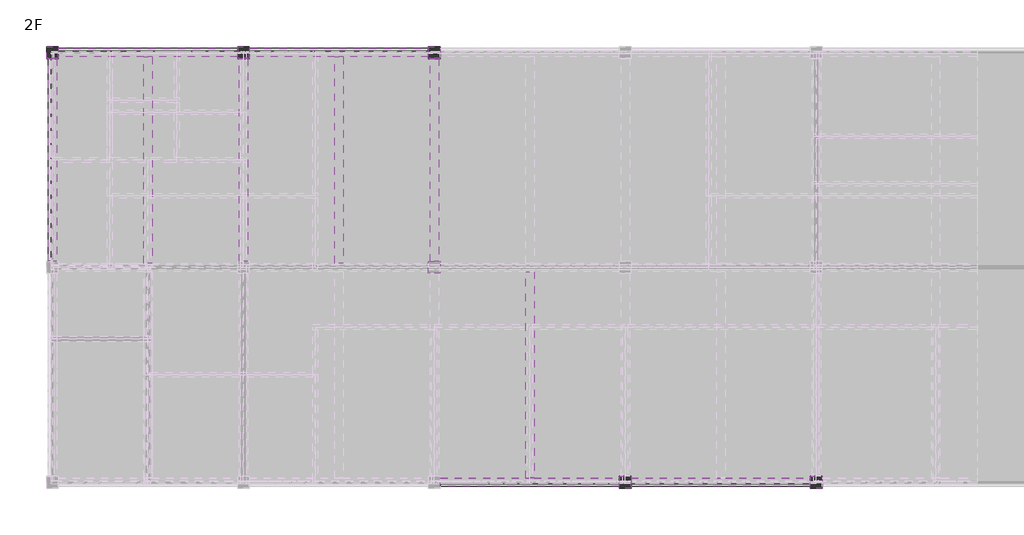
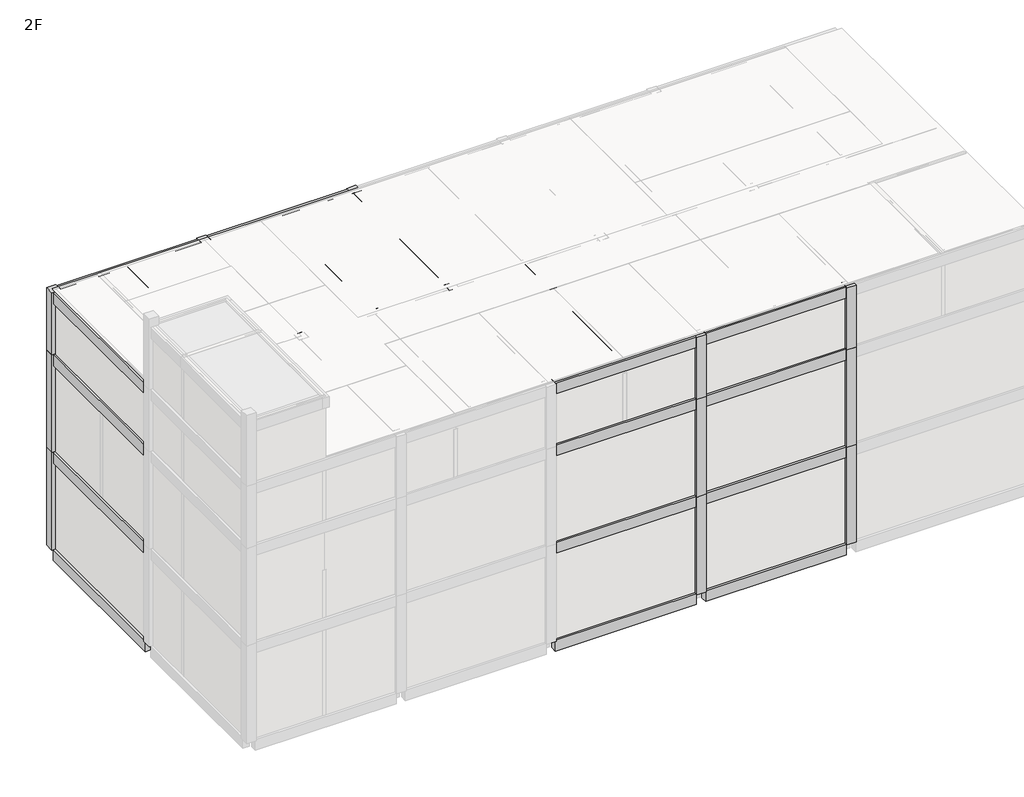
# One storey, part 5 of 7: 40 beams, 17 columns.
"""IFC4 building model written with IfcOpenShell, lengths in millimetres."""

from ifc_helpers import new_model, si_unit, frame, origin, place, context, project, spatial, polyline, outline, extrude, faceted_brep, element, save

model = new_model("IFC4")

# Units and contexts
model_context = context("Model", 3, world=origin())
ifc_project = project(units=[si_unit("LENGTHUNIT", "METRE", prefix="MILLI")], contexts=[model_context])

# Site, building, storey
site = spatial("IfcSite", under=ifc_project)
building = spatial("IfcBuilding", under=site)
storey = spatial("IfcBuildingStorey", under=building, Name="2F", Elevation=3500.0)

# Beams
placement = place(None, origin())
element("IfcBeam", 1, ObjectType="Concrete-Rectangular-Beam : BM111_400x500_RG1", at=placement, inside=storey, context=model_context, shape_type="SweptSolid", body=[
    extrude(outline(polyline([(49284.6521483, 181748.8614395), (49634.6521483, 181748.8614395), (49634.6521483, 173098.8614395), (49284.6521483, 173098.8614395), (49284.6521483, 181748.8614395)])), frame((0.0, 0.0, 2900.0), z_axis=(0.0, 0.0, 1.0), x_axis=(1.0, 0.0, 0.0)), (0.0, 0.0, 1.0), 600.0),
])
element("IfcBeam", 2, ObjectType="Concrete-Rectangular-Beam : BM111_400x500_RG1", at=placement, inside=storey, context=model_context, shape_type="SweptSolid", body=[
    extrude(outline(polyline([(57634.6521483, 173098.8614395), (57284.6521483, 173098.8614395), (57284.6521483, 181748.8614395), (57634.6521483, 181748.8614395), (57634.6521483, 173098.8614395)])), frame((0.0, 0.0, 2900.0), z_axis=(0.0, 0.0, 1.0), x_axis=(1.0, 0.0, 0.0)), (0.0, 0.0, 1.0), 600.0),
])
element("IfcBeam", 3, ObjectType="Concrete-Rectangular-Beam : BM111_400x500_RG1", at=placement, inside=storey, context=model_context, shape_type="SweptSolid", body=[
    extrude(outline(polyline([(65284.6521483, 172748.8614395), (65634.6521483, 172748.8614395), (65634.6521483, 164098.8614395), (65284.6521483, 164098.8614395), (65284.6521483, 172748.8614395)])), frame((0.0, 0.0, 2900.0), z_axis=(0.0, 0.0, 1.0), x_axis=(1.0, 0.0, 0.0)), (0.0, 0.0, 1.0), 600.0),
])
element("IfcBeam", 4, ObjectType="Concrete-Rectangular-Beam : BM111_400x500_RG1", at=placement, inside=storey, context=model_context, shape_type="SweptSolid", body=[
    extrude(outline(polyline([(49284.6521483, 181748.8614395), (49634.6521483, 181748.8614395), (49634.6521483, 173098.8614395), (49284.6521483, 173098.8614395), (49284.6521483, 181748.8614395)])), frame((0.0, 0.0, 8400.0), z_axis=(0.0, 0.0, 1.0), x_axis=(1.0, 0.0, 0.0)), (0.0, 0.0, 1.0), 600.0),
])
element("IfcBeam", 5, ObjectType="Concrete-Rectangular-Beam : BM111_400x500_RG1", at=placement, inside=storey, context=model_context, shape_type="SweptSolid", body=[
    extrude(outline(polyline([(57634.6521483, 173098.8614395), (57284.6521483, 173098.8614395), (57284.6521483, 181748.8614395), (57634.6521483, 181748.8614395), (57634.6521483, 173098.8614395)])), frame((0.0, 0.0, 8400.0), z_axis=(0.0, 0.0, 1.0), x_axis=(1.0, 0.0, 0.0)), (0.0, 0.0, 1.0), 600.0),
])
element("IfcBeam", 6, ObjectType="Concrete-Rectangular-Beam : BM111_400x500_RG1", at=placement, inside=storey, context=model_context, shape_type="SweptSolid", body=[
    extrude(outline(polyline([(65284.6521483, 172748.8614395), (65634.6521483, 172748.8614395), (65634.6521483, 164098.8614395), (65284.6521483, 164098.8614395), (65284.6521483, 172748.8614395)])), frame((0.0, 0.0, 8400.0), z_axis=(0.0, 0.0, 1.0), x_axis=(1.0, 0.0, 0.0)), (0.0, 0.0, 1.0), 600.0),
])
element("IfcBeam", 7, ObjectType="Concrete-Rectangular-Beam : BM111_400x500_RG1", at=placement, inside=storey, context=model_context, shape_type="SweptSolid", body=[
    extrude(outline(polyline([(49284.6521483, 181748.8614395), (49634.6521483, 181748.8614395), (49634.6521483, 173098.8614395), (49284.6521483, 173098.8614395), (49284.6521483, 181748.8614395)])), frame((0.0, 0.0, 13900.0), z_axis=(0.0, 0.0, 1.0), x_axis=(1.0, 0.0, 0.0)), (0.0, 0.0, 1.0), 600.0),
])
element("IfcBeam", 8, ObjectType="Concrete-Rectangular-Beam : BM111_400x500_RG1", at=placement, inside=storey, context=model_context, shape_type="SweptSolid", body=[
    extrude(outline(polyline([(57634.6521483, 173098.8614395), (57284.6521483, 173098.8614395), (57284.6521483, 181748.8614395), (57634.6521483, 181748.8614395), (57634.6521483, 173098.8614395)])), frame((0.0, 0.0, 13900.0), z_axis=(0.0, 0.0, 1.0), x_axis=(1.0, 0.0, 0.0)), (0.0, 0.0, 1.0), 600.0),
])
element("IfcBeam", 9, ObjectType="Concrete-Rectangular-Beam : BM111_400x500_RG1", at=placement, inside=storey, context=model_context, shape_type="SweptSolid", body=[
    extrude(outline(polyline([(65284.6521483, 172748.8614395), (65634.6521483, 172748.8614395), (65634.6521483, 164098.8614395), (65284.6521483, 164098.8614395), (65284.6521483, 172748.8614395)])), frame((0.0, 0.0, 13900.0), z_axis=(0.0, 0.0, 1.0), x_axis=(1.0, 0.0, 0.0)), (0.0, 0.0, 1.0), 600.0),
])
element("IfcBeam", 10, ObjectType="Concrete-Rectangular-Beam : BM111_400x500_RG1", at=placement, inside=storey, context=model_context, shape_type="SweptSolid", body=[
    extrude(outline(polyline([(49284.6521483, 181748.8614395), (49634.6521483, 181748.8614395), (49634.6521483, 173098.8614395), (49284.6521483, 173098.8614395), (49284.6521483, 181748.8614395)])), frame((0.0, 0.0, 17400.0), z_axis=(0.0, 0.0, 1.0), x_axis=(1.0, 0.0, 0.0)), (0.0, 0.0, 1.0), 600.0),
])
element("IfcBeam", 11, ObjectType="Concrete-Rectangular-Beam : BM111_400x500_RG1", at=placement, inside=storey, context=model_context, shape_type="SweptSolid", body=[
    extrude(outline(polyline([(57634.6521483, 173098.8614395), (57284.6521483, 173098.8614395), (57284.6521483, 181748.8614395), (57634.6521483, 181748.8614395), (57634.6521483, 173098.8614395)])), frame((0.0, 0.0, 17400.0), z_axis=(0.0, 0.0, 1.0), x_axis=(1.0, 0.0, 0.0)), (0.0, 0.0, 1.0), 600.0),
])
element("IfcBeam", 12, ObjectType="Concrete-Rectangular-Beam : BM111_400x500_RG1", at=placement, inside=storey, context=model_context, shape_type="SweptSolid", body=[
    extrude(outline(polyline([(65284.6521483, 172748.8614395), (65634.6521483, 172748.8614395), (65634.6521483, 164098.8614395), (65284.6521483, 164098.8614395), (65284.6521483, 172748.8614395)])), frame((0.0, 0.0, 17400.0), z_axis=(0.0, 0.0, 1.0), x_axis=(1.0, 0.0, 0.0)), (0.0, 0.0, 1.0), 600.0),
])
element("IfcBeam", 13, ObjectType="Concrete-Rectangular-Beam : BM111_400x500_RG1", at=placement, inside=storey, context=model_context, shape_type="Brep", body=[
    faceted_brep([(45709.6521483, 182098.8614395, 3500.0), (45709.6521483, 181748.8614395, 3500.0), (49284.6521483, 181748.8614395, 3500.0), (49634.6521483, 181748.8614395, 3500.0), (53209.6521483, 181748.8614395, 3500.0), (53209.6521483, 182098.8614395, 3500.0), (45709.6521483, 181748.8614395, 2900.0), (49284.6521483, 181748.8614395, 2900.0), (49634.6521483, 181748.8614395, 2900.0), (53209.6521483, 181748.8614395, 2900.0), (45709.6521483, 182098.8614395, 2900.0), (53209.6521483, 182098.8614395, 2900.0)], [[[0, 1, 2, 3, 4, 5]], [[1, 6, 7, 8, 9, 4, 3, 2]], [[6, 10, 11, 9, 8, 7]], [[10, 0, 5, 11]], [[1, 0, 10, 6]], [[5, 4, 9, 11]]]),
])
element("IfcBeam", 14, ObjectType="Concrete-Rectangular-Beam : BM111_400x500_RG1", at=placement, inside=storey, context=model_context, shape_type="Brep", body=[
    faceted_brep([(53709.6521483, 182098.8614395, 3500.0), (53709.6521483, 181748.8614395, 3500.0), (57284.6521483, 181748.8614395, 3500.0), (57634.6521483, 181748.8614395, 3500.0), (61209.6521483, 181748.8614395, 3500.0), (61209.6521483, 182098.8614395, 3500.0), (53709.6521483, 181748.8614395, 2900.0), (57284.6521483, 181748.8614395, 2900.0), (57634.6521483, 181748.8614395, 2900.0), (61209.6521483, 181748.8614395, 2900.0), (53709.6521483, 182098.8614395, 2900.0), (61209.6521483, 182098.8614395, 2900.0)], [[[0, 1, 2, 3, 4, 5]], [[1, 6, 7, 8, 9, 4, 3, 2]], [[6, 10, 11, 9, 8, 7]], [[10, 0, 5, 11]], [[1, 0, 10, 6]], [[5, 4, 9, 11]]]),
])
element("IfcBeam", 15, ObjectType="Concrete-Rectangular-Beam : BM111_400x500_RG1", at=placement, inside=storey, context=model_context, shape_type="Brep", body=[
    faceted_brep([(61709.6521483, 164098.8614395, 3500.0), (61709.6521483, 163748.8614395, 3500.0), (69209.6521483, 163748.8614395, 3500.0), (69209.6521483, 164098.8614395, 3500.0), (65634.6521483, 164098.8614395, 3500.0), (65284.6521483, 164098.8614395, 3500.0), (61709.6521483, 163748.8614395, 2900.0), (69209.6521483, 163748.8614395, 2900.0), (61709.6521483, 164098.8614395, 2900.0), (65284.6521483, 164098.8614395, 2900.0), (65634.6521483, 164098.8614395, 2900.0), (69209.6521483, 164098.8614395, 2900.0)], [[[0, 1, 2, 3, 4, 5]], [[1, 6, 7, 2]], [[6, 8, 9, 10, 11, 7]], [[8, 0, 5, 4, 3, 11, 10, 9]], [[1, 0, 8, 6]], [[3, 2, 7, 11]]]),
])
element("IfcBeam", 16, ObjectType="Concrete-Rectangular-Beam : BM111_400x500_RG1", at=placement, inside=storey, context=model_context, shape_type="Brep", body=[
    faceted_brep([(69709.6521483, 164098.8614395, 3500.0), (69709.6521483, 163748.8614395, 3500.0), (77209.6521483, 163748.8614395, 3500.0), (77209.6521483, 164098.8614395, 3500.0), (73634.6521483, 164098.8614395, 3500.0), (73284.6521483, 164098.8614395, 3500.0), (69709.6521483, 163748.8614395, 2900.0), (77209.6521483, 163748.8614395, 2900.0), (69709.6521483, 164098.8614395, 2900.0), (73284.6521483, 164098.8614395, 2900.0), (73634.6521483, 164098.8614395, 2900.0), (77209.6521483, 164098.8614395, 2900.0)], [[[0, 1, 2, 3, 4, 5]], [[1, 6, 7, 2]], [[6, 8, 9, 10, 11, 7]], [[8, 0, 5, 4, 3, 11, 10, 9]], [[1, 0, 8, 6]], [[3, 2, 7, 11]]]),
])
element("IfcBeam", 17, ObjectType="Concrete-Rectangular-Beam : BM111_400x500_RG1", at=placement, inside=storey, context=model_context, shape_type="Brep", body=[
    faceted_brep([(45709.6521483, 182098.8614395, 9000.0), (45709.6521483, 181748.8614395, 9000.0), (49284.6521483, 181748.8614395, 9000.0), (49634.6521483, 181748.8614395, 9000.0), (53209.6521483, 181748.8614395, 9000.0), (53209.6521483, 182098.8614395, 9000.0), (45709.6521483, 181748.8614395, 8400.0), (49284.6521483, 181748.8614395, 8400.0), (49634.6521483, 181748.8614395, 8400.0), (53209.6521483, 181748.8614395, 8400.0), (45709.6521483, 182098.8614395, 8400.0), (53209.6521483, 182098.8614395, 8400.0)], [[[0, 1, 2, 3, 4, 5]], [[1, 6, 7, 8, 9, 4, 3, 2]], [[6, 10, 11, 9, 8, 7]], [[10, 0, 5, 11]], [[1, 0, 10, 6]], [[5, 4, 9, 11]]]),
])
element("IfcBeam", 18, ObjectType="Concrete-Rectangular-Beam : BM111_400x500_RG1", at=placement, inside=storey, context=model_context, shape_type="Brep", body=[
    faceted_brep([(53709.6521483, 182098.8614395, 9000.0), (53709.6521483, 181748.8614395, 9000.0), (57284.6521483, 181748.8614395, 9000.0), (57634.6521483, 181748.8614395, 9000.0), (61209.6521483, 181748.8614395, 9000.0), (61209.6521483, 182098.8614395, 9000.0), (53709.6521483, 181748.8614395, 8400.0), (57284.6521483, 181748.8614395, 8400.0), (57634.6521483, 181748.8614395, 8400.0), (61209.6521483, 181748.8614395, 8400.0), (53709.6521483, 182098.8614395, 8400.0), (61209.6521483, 182098.8614395, 8400.0)], [[[0, 1, 2, 3, 4, 5]], [[1, 6, 7, 8, 9, 4, 3, 2]], [[6, 10, 11, 9, 8, 7]], [[10, 0, 5, 11]], [[1, 0, 10, 6]], [[5, 4, 9, 11]]]),
])
element("IfcBeam", 19, ObjectType="Concrete-Rectangular-Beam : BM111_400x500_RG1", at=placement, inside=storey, context=model_context, shape_type="Brep", body=[
    faceted_brep([(61709.6521483, 164098.8614395, 9000.0), (61709.6521483, 163748.8614395, 9000.0), (69209.6521483, 163748.8614395, 9000.0), (69209.6521483, 164098.8614395, 9000.0), (65634.6521483, 164098.8614395, 9000.0), (65284.6521483, 164098.8614395, 9000.0), (61709.6521483, 163748.8614395, 8400.0), (69209.6521483, 163748.8614395, 8400.0), (61709.6521483, 164098.8614395, 8400.0), (65284.6521483, 164098.8614395, 8400.0), (65634.6521483, 164098.8614395, 8400.0), (69209.6521483, 164098.8614395, 8400.0)], [[[0, 1, 2, 3, 4, 5]], [[1, 6, 7, 2]], [[6, 8, 9, 10, 11, 7]], [[8, 0, 5, 4, 3, 11, 10, 9]], [[1, 0, 8, 6]], [[3, 2, 7, 11]]]),
])
element("IfcBeam", 20, ObjectType="Concrete-Rectangular-Beam : BM111_400x500_RG1", at=placement, inside=storey, context=model_context, shape_type="Brep", body=[
    faceted_brep([(69709.6521483, 164098.8614395, 9000.0), (69709.6521483, 163748.8614395, 9000.0), (77209.6521483, 163748.8614395, 9000.0), (77209.6521483, 164098.8614395, 9000.0), (73634.6521483, 164098.8614395, 9000.0), (73284.6521483, 164098.8614395, 9000.0), (69709.6521483, 163748.8614395, 8400.0), (77209.6521483, 163748.8614395, 8400.0), (69709.6521483, 164098.8614395, 8400.0), (73284.6521483, 164098.8614395, 8400.0), (73634.6521483, 164098.8614395, 8400.0), (77209.6521483, 164098.8614395, 8400.0)], [[[0, 1, 2, 3, 4, 5]], [[1, 6, 7, 2]], [[6, 8, 9, 10, 11, 7]], [[8, 0, 5, 4, 3, 11, 10, 9]], [[1, 0, 8, 6]], [[3, 2, 7, 11]]]),
])
element("IfcBeam", 21, ObjectType="Concrete-Rectangular-Beam : BM111_400x500_RG1", at=placement, inside=storey, context=model_context, shape_type="Brep", body=[
    faceted_brep([(45709.6521483, 182098.8614395, 14500.0), (45709.6521483, 181748.8614395, 14500.0), (49284.6521483, 181748.8614395, 14500.0), (49634.6521483, 181748.8614395, 14500.0), (53209.6521483, 181748.8614395, 14500.0), (53209.6521483, 182098.8614395, 14500.0), (45709.6521483, 181748.8614395, 13900.0), (49284.6521483, 181748.8614395, 13900.0), (49634.6521483, 181748.8614395, 13900.0), (53209.6521483, 181748.8614395, 13900.0), (45709.6521483, 182098.8614395, 13900.0), (53209.6521483, 182098.8614395, 13900.0)], [[[0, 1, 2, 3, 4, 5]], [[1, 6, 7, 8, 9, 4, 3, 2]], [[6, 10, 11, 9, 8, 7]], [[10, 0, 5, 11]], [[1, 0, 10, 6]], [[5, 4, 9, 11]]]),
])
element("IfcBeam", 22, ObjectType="Concrete-Rectangular-Beam : BM111_400x500_RG1", at=placement, inside=storey, context=model_context, shape_type="Brep", body=[
    faceted_brep([(53709.6521483, 182098.8614395, 14500.0), (53709.6521483, 181748.8614395, 14500.0), (57284.6521483, 181748.8614395, 14500.0), (57634.6521483, 181748.8614395, 14500.0), (61209.6521483, 181748.8614395, 14500.0), (61209.6521483, 182098.8614395, 14500.0), (53709.6521483, 181748.8614395, 13900.0), (57284.6521483, 181748.8614395, 13900.0), (57634.6521483, 181748.8614395, 13900.0), (61209.6521483, 181748.8614395, 13900.0), (53709.6521483, 182098.8614395, 13900.0), (61209.6521483, 182098.8614395, 13900.0)], [[[0, 1, 2, 3, 4, 5]], [[1, 6, 7, 8, 9, 4, 3, 2]], [[6, 10, 11, 9, 8, 7]], [[10, 0, 5, 11]], [[1, 0, 10, 6]], [[5, 4, 9, 11]]]),
])
element("IfcBeam", 23, ObjectType="Concrete-Rectangular-Beam : BM111_400x500_RG1", at=placement, inside=storey, context=model_context, shape_type="Brep", body=[
    faceted_brep([(61709.6521483, 164098.8614395, 14500.0), (61709.6521483, 163748.8614395, 14500.0), (69209.6521483, 163748.8614395, 14500.0), (69209.6521483, 164098.8614395, 14500.0), (65634.6521483, 164098.8614395, 14500.0), (65284.6521483, 164098.8614395, 14500.0), (61709.6521483, 163748.8614395, 13900.0), (69209.6521483, 163748.8614395, 13900.0), (61709.6521483, 164098.8614395, 13900.0), (65284.6521483, 164098.8614395, 13900.0), (65634.6521483, 164098.8614395, 13900.0), (69209.6521483, 164098.8614395, 13900.0)], [[[0, 1, 2, 3, 4, 5]], [[1, 6, 7, 2]], [[6, 8, 9, 10, 11, 7]], [[8, 0, 5, 4, 3, 11, 10, 9]], [[1, 0, 8, 6]], [[3, 2, 7, 11]]]),
])
element("IfcBeam", 24, ObjectType="Concrete-Rectangular-Beam : BM111_400x500_RG1", at=placement, inside=storey, context=model_context, shape_type="Brep", body=[
    faceted_brep([(69709.6521483, 164098.8614395, 14500.0), (69709.6521483, 163748.8614395, 14500.0), (77209.6521483, 163748.8614395, 14500.0), (77209.6521483, 164098.8614395, 14500.0), (73634.6521483, 164098.8614395, 14500.0), (73284.6521483, 164098.8614395, 14500.0), (69709.6521483, 163748.8614395, 13900.0), (77209.6521483, 163748.8614395, 13900.0), (69709.6521483, 164098.8614395, 13900.0), (73284.6521483, 164098.8614395, 13900.0), (73634.6521483, 164098.8614395, 13900.0), (77209.6521483, 164098.8614395, 13900.0)], [[[0, 1, 2, 3, 4, 5]], [[1, 6, 7, 2]], [[6, 8, 9, 10, 11, 7]], [[8, 0, 5, 4, 3, 11, 10, 9]], [[1, 0, 8, 6]], [[3, 2, 7, 11]]]),
])
element("IfcBeam", 25, ObjectType="Concrete-Rectangular-Beam : BM111_400x500_RG1", at=placement, inside=storey, context=model_context, shape_type="Brep", body=[
    faceted_brep([(45709.6521483, 182098.8614395, 18000.0), (45709.6521483, 181748.8614395, 18000.0), (49284.6521483, 181748.8614395, 18000.0), (49634.6521483, 181748.8614395, 18000.0), (53209.6521483, 181748.8614395, 18000.0), (53209.6521483, 182098.8614395, 18000.0), (45709.6521483, 181748.8614395, 17400.0), (49284.6521483, 181748.8614395, 17400.0), (49634.6521483, 181748.8614395, 17400.0), (53209.6521483, 181748.8614395, 17400.0), (45709.6521483, 182098.8614395, 17400.0), (53209.6521483, 182098.8614395, 17400.0)], [[[0, 1, 2, 3, 4, 5]], [[1, 6, 7, 8, 9, 4, 3, 2]], [[6, 10, 11, 9, 8, 7]], [[10, 0, 5, 11]], [[1, 0, 10, 6]], [[5, 4, 9, 11]]]),
])
element("IfcBeam", 26, ObjectType="Concrete-Rectangular-Beam : BM111_400x500_RG1", at=placement, inside=storey, context=model_context, shape_type="Brep", body=[
    faceted_brep([(53709.6521483, 182098.8614395, 18000.0), (53709.6521483, 181748.8614395, 18000.0), (57284.6521483, 181748.8614395, 18000.0), (57634.6521483, 181748.8614395, 18000.0), (61209.6521483, 181748.8614395, 18000.0), (61209.6521483, 182098.8614395, 18000.0), (53709.6521483, 181748.8614395, 17400.0), (57284.6521483, 181748.8614395, 17400.0), (57634.6521483, 181748.8614395, 17400.0), (61209.6521483, 181748.8614395, 17400.0), (53709.6521483, 182098.8614395, 17400.0), (61209.6521483, 182098.8614395, 17400.0)], [[[0, 1, 2, 3, 4, 5]], [[1, 6, 7, 8, 9, 4, 3, 2]], [[6, 10, 11, 9, 8, 7]], [[10, 0, 5, 11]], [[1, 0, 10, 6]], [[5, 4, 9, 11]]]),
])
element("IfcBeam", 27, ObjectType="Concrete-Rectangular-Beam : BM111_400x500_RG1", at=placement, inside=storey, context=model_context, shape_type="Brep", body=[
    faceted_brep([(61709.6521483, 164098.8614395, 18000.0), (61709.6521483, 163748.8614395, 18000.0), (69209.6521483, 163748.8614395, 18000.0), (69209.6521483, 164098.8614395, 18000.0), (65634.6521483, 164098.8614395, 18000.0), (65284.6521483, 164098.8614395, 18000.0), (61709.6521483, 163748.8614395, 17400.0), (69209.6521483, 163748.8614395, 17400.0), (61709.6521483, 164098.8614395, 17400.0), (65284.6521483, 164098.8614395, 17400.0), (65634.6521483, 164098.8614395, 17400.0), (69209.6521483, 164098.8614395, 17400.0)], [[[0, 1, 2, 3, 4, 5]], [[1, 6, 7, 2]], [[6, 8, 9, 10, 11, 7]], [[8, 0, 5, 4, 3, 11, 10, 9]], [[1, 0, 8, 6]], [[3, 2, 7, 11]]]),
])
element("IfcBeam", 28, ObjectType="Concrete-Rectangular-Beam : BM111_400x500_RG1", at=placement, inside=storey, context=model_context, shape_type="Brep", body=[
    faceted_brep([(69709.6521483, 164098.8614395, 18000.0), (69709.6521483, 163748.8614395, 18000.0), (77209.6521483, 163748.8614395, 18000.0), (77209.6521483, 164098.8614395, 18000.0), (73634.6521483, 164098.8614395, 18000.0), (73284.6521483, 164098.8614395, 18000.0), (69709.6521483, 163748.8614395, 17400.0), (77209.6521483, 163748.8614395, 17400.0), (69709.6521483, 164098.8614395, 17400.0), (73284.6521483, 164098.8614395, 17400.0), (73634.6521483, 164098.8614395, 17400.0), (77209.6521483, 164098.8614395, 17400.0)], [[[0, 1, 2, 3, 4, 5]], [[1, 6, 7, 2]], [[6, 8, 9, 10, 11, 7]], [[8, 0, 5, 4, 3, 11, 10, 9]], [[1, 0, 8, 6]], [[3, 2, 7, 11]]]),
])
element("IfcBeam", 29, ObjectType="Concrete-Rectangular-Beam : BM111_400x500_RG1", at=placement, inside=storey, context=model_context, shape_type="SweptSolid", body=[
    extrude(outline(polyline([(45284.6521483, 181673.8614395), (45634.6521483, 181673.8614395), (45634.6521483, 173173.8614395), (45284.6521483, 173173.8614395), (45284.6521483, 181673.8614395)])), frame((0.0, 0.0, 2900.0), z_axis=(0.0, 0.0, 1.0), x_axis=(1.0, 0.0, 0.0)), (0.0, 0.0, 1.0), 600.0),
])
element("IfcBeam", 30, ObjectType="Concrete-Rectangular-Beam : BM111_400x500_RG1", at=placement, inside=storey, context=model_context, shape_type="SweptSolid", body=[
    extrude(outline(polyline([(53284.6521483, 181673.8614395), (53634.6521483, 181673.8614395), (53634.6521483, 173173.8614395), (53284.6521483, 173173.8614395), (53284.6521483, 181673.8614395)])), frame((0.0, 0.0, 2900.0), z_axis=(0.0, 0.0, 1.0), x_axis=(1.0, 0.0, 0.0)), (0.0, 0.0, 1.0), 600.0),
])
element("IfcBeam", 31, ObjectType="Concrete-Rectangular-Beam : BM111_400x500_RG1", at=placement, inside=storey, context=model_context, shape_type="SweptSolid", body=[
    extrude(outline(polyline([(61284.6521483, 181673.8614395), (61634.6521483, 181673.8614395), (61634.6521483, 173173.8614395), (61284.6521483, 173173.8614395), (61284.6521483, 181673.8614395)])), frame((0.0, 0.0, 2900.0), z_axis=(0.0, 0.0, 1.0), x_axis=(1.0, 0.0, 0.0)), (0.0, 0.0, 1.0), 600.0),
])
element("IfcBeam", 32, ObjectType="Concrete-Rectangular-Beam : BM111_400x500_RG1", at=placement, inside=storey, context=model_context, shape_type="SweptSolid", body=[
    extrude(outline(polyline([(45284.6521483, 181673.8614395), (45634.6521483, 181673.8614395), (45634.6521483, 173173.8614395), (45284.6521483, 173173.8614395), (45284.6521483, 181673.8614395)])), frame((0.0, 0.0, 8400.0), z_axis=(0.0, 0.0, 1.0), x_axis=(1.0, 0.0, 0.0)), (0.0, 0.0, 1.0), 600.0),
])
element("IfcBeam", 33, ObjectType="Concrete-Rectangular-Beam : BM111_400x500_RG1", at=placement, inside=storey, context=model_context, shape_type="SweptSolid", body=[
    extrude(outline(polyline([(53284.6521483, 181673.8614395), (53634.6521483, 181673.8614395), (53634.6521483, 173173.8614395), (53284.6521483, 173173.8614395), (53284.6521483, 181673.8614395)])), frame((0.0, 0.0, 8400.0), z_axis=(0.0, 0.0, 1.0), x_axis=(1.0, 0.0, 0.0)), (0.0, 0.0, 1.0), 600.0),
])
element("IfcBeam", 34, ObjectType="Concrete-Rectangular-Beam : BM111_400x500_RG1", at=placement, inside=storey, context=model_context, shape_type="SweptSolid", body=[
    extrude(outline(polyline([(61284.6521483, 181673.8614395), (61634.6521483, 181673.8614395), (61634.6521483, 173173.8614395), (61284.6521483, 173173.8614395), (61284.6521483, 181673.8614395)])), frame((0.0, 0.0, 8400.0), z_axis=(0.0, 0.0, 1.0), x_axis=(1.0, 0.0, 0.0)), (0.0, 0.0, 1.0), 600.0),
])
element("IfcBeam", 35, ObjectType="Concrete-Rectangular-Beam : BM111_400x500_RG1", at=placement, inside=storey, context=model_context, shape_type="SweptSolid", body=[
    extrude(outline(polyline([(45284.6521483, 181673.8614395), (45634.6521483, 181673.8614395), (45634.6521483, 173173.8614395), (45284.6521483, 173173.8614395), (45284.6521483, 181673.8614395)])), frame((0.0, 0.0, 13900.0), z_axis=(0.0, 0.0, 1.0), x_axis=(1.0, 0.0, 0.0)), (0.0, 0.0, 1.0), 600.0),
])
element("IfcBeam", 36, ObjectType="Concrete-Rectangular-Beam : BM111_400x500_RG1", at=placement, inside=storey, context=model_context, shape_type="SweptSolid", body=[
    extrude(outline(polyline([(53284.6521483, 181673.8614395), (53634.6521483, 181673.8614395), (53634.6521483, 173173.8614395), (53284.6521483, 173173.8614395), (53284.6521483, 181673.8614395)])), frame((0.0, 0.0, 13900.0), z_axis=(0.0, 0.0, 1.0), x_axis=(1.0, 0.0, 0.0)), (0.0, 0.0, 1.0), 600.0),
])
element("IfcBeam", 37, ObjectType="Concrete-Rectangular-Beam : BM111_400x500_RG1", at=placement, inside=storey, context=model_context, shape_type="SweptSolid", body=[
    extrude(outline(polyline([(61284.6521483, 181673.8614395), (61634.6521483, 181673.8614395), (61634.6521483, 173173.8614395), (61284.6521483, 173173.8614395), (61284.6521483, 181673.8614395)])), frame((0.0, 0.0, 13900.0), z_axis=(0.0, 0.0, 1.0), x_axis=(1.0, 0.0, 0.0)), (0.0, 0.0, 1.0), 600.0),
])
element("IfcBeam", 38, ObjectType="Concrete-Rectangular-Beam : BM111_400x500_RG1", at=placement, inside=storey, context=model_context, shape_type="SweptSolid", body=[
    extrude(outline(polyline([(45284.6521483, 181673.8614395), (45634.6521483, 181673.8614395), (45634.6521483, 173173.8614395), (45284.6521483, 173173.8614395), (45284.6521483, 181673.8614395)])), frame((0.0, 0.0, 17400.0), z_axis=(0.0, 0.0, 1.0), x_axis=(1.0, 0.0, 0.0)), (0.0, 0.0, 1.0), 600.0),
])
element("IfcBeam", 39, ObjectType="Concrete-Rectangular-Beam : BM111_400x500_RG1", at=placement, inside=storey, context=model_context, shape_type="SweptSolid", body=[
    extrude(outline(polyline([(53284.6521483, 181673.8614395), (53634.6521483, 181673.8614395), (53634.6521483, 173173.8614395), (53284.6521483, 173173.8614395), (53284.6521483, 181673.8614395)])), frame((0.0, 0.0, 17400.0), z_axis=(0.0, 0.0, 1.0), x_axis=(1.0, 0.0, 0.0)), (0.0, 0.0, 1.0), 600.0),
])
element("IfcBeam", 40, ObjectType="Concrete-Rectangular-Beam : BM111_400x500_RG1", at=placement, inside=storey, context=model_context, shape_type="SweptSolid", body=[
    extrude(outline(polyline([(61284.6521483, 181673.8614395), (61634.6521483, 181673.8614395), (61634.6521483, 173173.8614395), (61284.6521483, 173173.8614395), (61284.6521483, 181673.8614395)])), frame((0.0, 0.0, 17400.0), z_axis=(0.0, 0.0, 1.0), x_axis=(1.0, 0.0, 0.0)), (0.0, 0.0, 1.0), 600.0),
])

# Columns
element("IfcColumn", 41, ObjectType="Concrete-Rectangular-Column : CL111_500x500", at=placement, inside=storey, context=model_context, shape_type="Brep", body=[
    faceted_brep([(45709.6521483, 182173.8614395, 3500.0), (45709.6521483, 181673.8614395, 3500.0), (45209.6521483, 181673.8614395, 3500.0), (45209.6521483, 182173.8614395, 3500.0), (45709.6521483, 182173.8614395, 9000.0), (45709.6521483, 182098.8614395, 9000.0), (45709.6521483, 181748.8614395, 9000.0), (45709.6521483, 181673.8614395, 9000.0), (45634.6521483, 181673.8614395, 9000.0), (45284.6521483, 181673.8614395, 9000.0), (45209.6521483, 181673.8614395, 9000.0), (45209.6521483, 182173.8614395, 9000.0)], [[[0, 1, 2, 3]], [[4, 5, 6, 7, 1, 0]], [[7, 8, 9, 10, 2, 1]], [[10, 11, 3, 2]], [[11, 4, 0, 3]], [[4, 11, 10, 9, 8, 7, 6, 5]]]),
])
element("IfcColumn", 42, ObjectType="Concrete-Rectangular-Column : CL111_500x500", at=placement, inside=storey, context=model_context, shape_type="Brep", body=[
    faceted_brep([(45709.6521483, 182173.8614395, 9000.0), (45709.6521483, 181673.8614395, 9000.0), (45209.6521483, 181673.8614395, 9000.0), (45209.6521483, 182173.8614395, 9000.0), (45709.6521483, 182173.8614395, 14500.0), (45709.6521483, 182098.8614395, 14500.0), (45709.6521483, 181748.8614395, 14500.0), (45709.6521483, 181673.8614395, 14500.0), (45634.6521483, 181673.8614395, 14500.0), (45284.6521483, 181673.8614395, 14500.0), (45209.6521483, 181673.8614395, 14500.0), (45209.6521483, 182173.8614395, 14500.0)], [[[0, 1, 2, 3]], [[4, 5, 6, 7, 1, 0]], [[7, 8, 9, 10, 2, 1]], [[10, 11, 3, 2]], [[11, 4, 0, 3]], [[4, 11, 10, 9, 8, 7, 6, 5]]]),
])
element("IfcColumn", 43, ObjectType="Concrete-Rectangular-Column : CL111_500x500", at=placement, inside=storey, context=model_context, shape_type="Brep", body=[
    faceted_brep([(45709.6521483, 182173.8614395, 14500.0), (45709.6521483, 181673.8614395, 14500.0), (45209.6521483, 181673.8614395, 14500.0), (45209.6521483, 182173.8614395, 14500.0), (45709.6521483, 182173.8614395, 18000.0), (45709.6521483, 182098.8614395, 18000.0), (45709.6521483, 181748.8614395, 18000.0), (45709.6521483, 181673.8614395, 18000.0), (45634.6521483, 181673.8614395, 18000.0), (45284.6521483, 181673.8614395, 18000.0), (45209.6521483, 181673.8614395, 18000.0), (45209.6521483, 182173.8614395, 18000.0)], [[[0, 1, 2, 3]], [[4, 5, 6, 7, 1, 0]], [[7, 8, 9, 10, 2, 1]], [[10, 11, 3, 2]], [[11, 4, 0, 3]], [[4, 11, 10, 9, 8, 7, 6, 5]]]),
])
element("IfcColumn", 44, ObjectType="Concrete-Rectangular-Column : CL111_500x500", at=placement, inside=storey, context=model_context, shape_type="Brep", body=[
    faceted_brep([(53709.6521483, 182173.8614395, 3500.0), (53709.6521483, 181673.8614395, 3500.0), (53209.6521483, 181673.8614395, 3500.0), (53209.6521483, 182173.8614395, 3500.0), (53709.6521483, 182173.8614395, 9000.0), (53709.6521483, 182098.8614395, 9000.0), (53709.6521483, 181748.8614395, 9000.0), (53709.6521483, 181673.8614395, 9000.0), (53634.6521483, 181673.8614395, 9000.0), (53284.6521483, 181673.8614395, 9000.0), (53209.6521483, 181673.8614395, 9000.0), (53209.6521483, 181748.8614395, 9000.0), (53209.6521483, 182098.8614395, 9000.0), (53209.6521483, 182173.8614395, 9000.0)], [[[0, 1, 2, 3]], [[4, 5, 6, 7, 1, 0]], [[7, 8, 9, 10, 2, 1]], [[10, 11, 12, 13, 3, 2]], [[13, 4, 0, 3]], [[4, 13, 12, 11, 10, 9, 8, 7, 6, 5]]]),
])
element("IfcColumn", 45, ObjectType="Concrete-Rectangular-Column : CL111_500x500", at=placement, inside=storey, context=model_context, shape_type="Brep", body=[
    faceted_brep([(53709.6521483, 182173.8614395, 9000.0), (53709.6521483, 181673.8614395, 9000.0), (53209.6521483, 181673.8614395, 9000.0), (53209.6521483, 182173.8614395, 9000.0), (53709.6521483, 182173.8614395, 14500.0), (53709.6521483, 182098.8614395, 14500.0), (53709.6521483, 181748.8614395, 14500.0), (53709.6521483, 181673.8614395, 14500.0), (53634.6521483, 181673.8614395, 14500.0), (53284.6521483, 181673.8614395, 14500.0), (53209.6521483, 181673.8614395, 14500.0), (53209.6521483, 181748.8614395, 14500.0), (53209.6521483, 182098.8614395, 14500.0), (53209.6521483, 182173.8614395, 14500.0)], [[[0, 1, 2, 3]], [[4, 5, 6, 7, 1, 0]], [[7, 8, 9, 10, 2, 1]], [[10, 11, 12, 13, 3, 2]], [[13, 4, 0, 3]], [[4, 13, 12, 11, 10, 9, 8, 7, 6, 5]]]),
])
element("IfcColumn", 46, ObjectType="Concrete-Rectangular-Column : CL111_500x500", at=placement, inside=storey, context=model_context, shape_type="Brep", body=[
    faceted_brep([(53709.6521483, 182173.8614395, 14500.0), (53709.6521483, 181673.8614395, 14500.0), (53209.6521483, 181673.8614395, 14500.0), (53209.6521483, 182173.8614395, 14500.0), (53709.6521483, 182173.8614395, 18000.0), (53709.6521483, 182098.8614395, 18000.0), (53709.6521483, 181748.8614395, 18000.0), (53709.6521483, 181673.8614395, 18000.0), (53634.6521483, 181673.8614395, 18000.0), (53284.6521483, 181673.8614395, 18000.0), (53209.6521483, 181673.8614395, 18000.0), (53209.6521483, 181748.8614395, 18000.0), (53209.6521483, 182098.8614395, 18000.0), (53209.6521483, 182173.8614395, 18000.0)], [[[0, 1, 2, 3]], [[4, 5, 6, 7, 1, 0]], [[7, 8, 9, 10, 2, 1]], [[10, 11, 12, 13, 3, 2]], [[13, 4, 0, 3]], [[4, 13, 12, 11, 10, 9, 8, 7, 6, 5]]]),
])
element("IfcColumn", 47, ObjectType="Concrete-Rectangular-Column : CL111_500x500", at=placement, inside=storey, context=model_context, shape_type="Brep", body=[
    faceted_brep([(61709.6521483, 182173.8614395, 3500.0), (61709.6521483, 181673.8614395, 3500.0), (61209.6521483, 181673.8614395, 3500.0), (61209.6521483, 182173.8614395, 3500.0), (61709.6521483, 182173.8614395, 9000.0), (61709.6521483, 182098.8614395, 9000.0), (61709.6521483, 181748.8614395, 9000.0), (61709.6521483, 181673.8614395, 9000.0), (61634.6521483, 181673.8614395, 9000.0), (61284.6521483, 181673.8614395, 9000.0), (61209.6521483, 181673.8614395, 9000.0), (61209.6521483, 181748.8614395, 9000.0), (61209.6521483, 182098.8614395, 9000.0), (61209.6521483, 182173.8614395, 9000.0)], [[[0, 1, 2, 3]], [[4, 5, 6, 7, 1, 0]], [[7, 8, 9, 10, 2, 1]], [[10, 11, 12, 13, 3, 2]], [[13, 4, 0, 3]], [[4, 13, 12, 11, 10, 9, 8, 7, 6, 5]]]),
])
element("IfcColumn", 48, ObjectType="Concrete-Rectangular-Column : CL111_500x500", at=placement, inside=storey, context=model_context, shape_type="Brep", body=[
    faceted_brep([(61709.6521483, 182173.8614395, 9000.0), (61709.6521483, 181673.8614395, 9000.0), (61209.6521483, 181673.8614395, 9000.0), (61209.6521483, 182173.8614395, 9000.0), (61709.6521483, 182173.8614395, 14500.0), (61709.6521483, 182098.8614395, 14500.0), (61709.6521483, 181748.8614395, 14500.0), (61709.6521483, 181673.8614395, 14500.0), (61634.6521483, 181673.8614395, 14500.0), (61284.6521483, 181673.8614395, 14500.0), (61209.6521483, 181673.8614395, 14500.0), (61209.6521483, 181748.8614395, 14500.0), (61209.6521483, 182098.8614395, 14500.0), (61209.6521483, 182173.8614395, 14500.0)], [[[0, 1, 2, 3]], [[4, 5, 6, 7, 1, 0]], [[7, 8, 9, 10, 2, 1]], [[10, 11, 12, 13, 3, 2]], [[13, 4, 0, 3]], [[4, 13, 12, 11, 10, 9, 8, 7, 6, 5]]]),
])
element("IfcColumn", 49, ObjectType="Concrete-Rectangular-Column : CL111_500x500", at=placement, inside=storey, context=model_context, shape_type="Brep", body=[
    faceted_brep([(61709.6521483, 182173.8614395, 14500.0), (61709.6521483, 181673.8614395, 14500.0), (61209.6521483, 181673.8614395, 14500.0), (61209.6521483, 182173.8614395, 14500.0), (61709.6521483, 182173.8614395, 18000.0), (61709.6521483, 182098.8614395, 18000.0), (61709.6521483, 181748.8614395, 18000.0), (61709.6521483, 181673.8614395, 18000.0), (61634.6521483, 181673.8614395, 18000.0), (61284.6521483, 181673.8614395, 18000.0), (61209.6521483, 181673.8614395, 18000.0), (61209.6521483, 181748.8614395, 18000.0), (61209.6521483, 182098.8614395, 18000.0), (61209.6521483, 182173.8614395, 18000.0)], [[[0, 1, 2, 3]], [[4, 5, 6, 7, 1, 0]], [[7, 8, 9, 10, 2, 1]], [[10, 11, 12, 13, 3, 2]], [[13, 4, 0, 3]], [[4, 13, 12, 11, 10, 9, 8, 7, 6, 5]]]),
])
element("IfcColumn", 50, ObjectType="Concrete-Rectangular-Column : CL111_500x500", at=placement, inside=storey, context=model_context, shape_type="Brep", body=[
    faceted_brep([(61709.6521483, 173173.8614395, 9000.0), (61709.6521483, 172673.8614395, 9000.0), (61209.6521483, 172673.8614395, 9000.0), (61209.6521483, 173173.8614395, 9000.0), (61709.6521483, 173173.8614395, 14500.0), (61709.6521483, 173098.8614395, 14500.0), (61709.6521483, 172748.8614395, 14500.0), (61709.6521483, 172673.8614395, 14500.0), (61634.6521483, 172673.8614395, 14500.0), (61284.6521483, 172673.8614395, 14500.0), (61209.6521483, 172673.8614395, 14500.0), (61209.6521483, 172748.8614395, 14500.0), (61209.6521483, 173098.8614395, 14500.0), (61209.6521483, 173173.8614395, 14500.0), (61284.6521483, 173173.8614395, 14500.0), (61634.6521483, 173173.8614395, 14500.0)], [[[0, 1, 2, 3]], [[4, 5, 6, 7, 1, 0]], [[7, 8, 9, 10, 2, 1]], [[10, 11, 12, 13, 3, 2]], [[13, 14, 15, 4, 0, 3]], [[4, 15, 14, 13, 12, 11, 10, 9, 8, 7, 6, 5]]]),
])
element("IfcColumn", 51, ObjectType="Concrete-Rectangular-Column : CL111_500x500", at=placement, inside=storey, context=model_context, shape_type="Brep", body=[
    faceted_brep([(61709.6521483, 173173.8614395, 14500.0), (61709.6521483, 172673.8614395, 14500.0), (61209.6521483, 172673.8614395, 14500.0), (61209.6521483, 173173.8614395, 14500.0), (61709.6521483, 173173.8614395, 18000.0), (61709.6521483, 173098.8614395, 18000.0), (61709.6521483, 172748.8614395, 18000.0), (61709.6521483, 172673.8614395, 18000.0), (61634.6521483, 172673.8614395, 18000.0), (61284.6521483, 172673.8614395, 18000.0), (61209.6521483, 172673.8614395, 18000.0), (61209.6521483, 172748.8614395, 18000.0), (61209.6521483, 173098.8614395, 18000.0), (61209.6521483, 173173.8614395, 18000.0), (61284.6521483, 173173.8614395, 18000.0), (61634.6521483, 173173.8614395, 18000.0)], [[[0, 1, 2, 3]], [[4, 5, 6, 7, 1, 0]], [[7, 8, 9, 10, 2, 1]], [[10, 11, 12, 13, 3, 2]], [[13, 14, 15, 4, 0, 3]], [[4, 15, 14, 13, 12, 11, 10, 9, 8, 7, 6, 5]]]),
])
element("IfcColumn", 52, ObjectType="Concrete-Rectangular-Column : CL111_500x500", at=placement, inside=storey, context=model_context, shape_type="Brep", body=[
    faceted_brep([(69709.6521483, 164173.8614395, 3500.0), (69709.6521483, 163673.8614395, 3500.0), (69209.6521483, 163673.8614395, 3500.0), (69209.6521483, 164173.8614395, 3500.0), (69709.6521483, 164173.8614395, 9000.0), (69709.6521483, 164098.8614395, 9000.0), (69709.6521483, 163748.8614395, 9000.0), (69709.6521483, 163673.8614395, 9000.0), (69209.6521483, 163673.8614395, 9000.0), (69209.6521483, 163748.8614395, 9000.0), (69209.6521483, 164098.8614395, 9000.0), (69209.6521483, 164173.8614395, 9000.0), (69284.6521483, 164173.8614395, 9000.0), (69634.6521483, 164173.8614395, 9000.0)], [[[0, 1, 2, 3]], [[4, 5, 6, 7, 1, 0]], [[7, 8, 2, 1]], [[8, 9, 10, 11, 3, 2]], [[11, 12, 13, 4, 0, 3]], [[4, 13, 12, 11, 10, 9, 8, 7, 6, 5]]]),
])
element("IfcColumn", 53, ObjectType="Concrete-Rectangular-Column : CL111_500x500", at=placement, inside=storey, context=model_context, shape_type="Brep", body=[
    faceted_brep([(69709.6521483, 164173.8614395, 9000.0), (69709.6521483, 163673.8614395, 9000.0), (69209.6521483, 163673.8614395, 9000.0), (69209.6521483, 164173.8614395, 9000.0), (69709.6521483, 164173.8614395, 14500.0), (69709.6521483, 164098.8614395, 14500.0), (69709.6521483, 163748.8614395, 14500.0), (69709.6521483, 163673.8614395, 14500.0), (69209.6521483, 163673.8614395, 14500.0), (69209.6521483, 163748.8614395, 14500.0), (69209.6521483, 164098.8614395, 14500.0), (69209.6521483, 164173.8614395, 14500.0), (69284.6521483, 164173.8614395, 14500.0), (69634.6521483, 164173.8614395, 14500.0)], [[[0, 1, 2, 3]], [[4, 5, 6, 7, 1, 0]], [[7, 8, 2, 1]], [[8, 9, 10, 11, 3, 2]], [[11, 12, 13, 4, 0, 3]], [[4, 13, 12, 11, 10, 9, 8, 7, 6, 5]]]),
])
element("IfcColumn", 54, ObjectType="Concrete-Rectangular-Column : CL111_500x500", at=placement, inside=storey, context=model_context, shape_type="Brep", body=[
    faceted_brep([(69709.6521483, 164173.8614395, 14500.0), (69709.6521483, 163673.8614395, 14500.0), (69209.6521483, 163673.8614395, 14500.0), (69209.6521483, 164173.8614395, 14500.0), (69709.6521483, 164173.8614395, 18000.0), (69709.6521483, 164098.8614395, 18000.0), (69709.6521483, 163748.8614395, 18000.0), (69709.6521483, 163673.8614395, 18000.0), (69209.6521483, 163673.8614395, 18000.0), (69209.6521483, 163748.8614395, 18000.0), (69209.6521483, 164098.8614395, 18000.0), (69209.6521483, 164173.8614395, 18000.0), (69284.6521483, 164173.8614395, 18000.0), (69634.6521483, 164173.8614395, 18000.0)], [[[0, 1, 2, 3]], [[4, 5, 6, 7, 1, 0]], [[7, 8, 2, 1]], [[8, 9, 10, 11, 3, 2]], [[11, 12, 13, 4, 0, 3]], [[4, 13, 12, 11, 10, 9, 8, 7, 6, 5]]]),
])
element("IfcColumn", 55, ObjectType="Concrete-Rectangular-Column : CL111_500x500", at=placement, inside=storey, context=model_context, shape_type="Brep", body=[
    faceted_brep([(77709.6521483, 164173.8614395, 3500.0), (77709.6521483, 163673.8614395, 3500.0), (77209.6521483, 163673.8614395, 3500.0), (77209.6521483, 164173.8614395, 3500.0), (77709.6521483, 164173.8614395, 9000.0), (77709.6521483, 164098.8614395, 9000.0), (77709.6521483, 163748.8614395, 9000.0), (77709.6521483, 163673.8614395, 9000.0), (77209.6521483, 163673.8614395, 9000.0), (77209.6521483, 163748.8614395, 9000.0), (77209.6521483, 164098.8614395, 9000.0), (77209.6521483, 164173.8614395, 9000.0), (77284.6521483, 164173.8614395, 9000.0), (77634.6521483, 164173.8614395, 9000.0)], [[[0, 1, 2, 3]], [[4, 5, 6, 7, 1, 0]], [[7, 8, 2, 1]], [[8, 9, 10, 11, 3, 2]], [[11, 12, 13, 4, 0, 3]], [[4, 13, 12, 11, 10, 9, 8, 7, 6, 5]]]),
])
element("IfcColumn", 56, ObjectType="Concrete-Rectangular-Column : CL111_500x500", at=placement, inside=storey, context=model_context, shape_type="Brep", body=[
    faceted_brep([(77709.6521483, 164173.8614395, 9000.0), (77709.6521483, 163673.8614395, 9000.0), (77209.6521483, 163673.8614395, 9000.0), (77209.6521483, 164173.8614395, 9000.0), (77709.6521483, 164173.8614395, 14500.0), (77709.6521483, 164098.8614395, 14500.0), (77709.6521483, 163748.8614395, 14500.0), (77709.6521483, 163673.8614395, 14500.0), (77209.6521483, 163673.8614395, 14500.0), (77209.6521483, 163748.8614395, 14500.0), (77209.6521483, 164098.8614395, 14500.0), (77209.6521483, 164173.8614395, 14500.0), (77284.6521483, 164173.8614395, 14500.0), (77634.6521483, 164173.8614395, 14500.0)], [[[0, 1, 2, 3]], [[4, 5, 6, 7, 1, 0]], [[7, 8, 2, 1]], [[8, 9, 10, 11, 3, 2]], [[11, 12, 13, 4, 0, 3]], [[4, 13, 12, 11, 10, 9, 8, 7, 6, 5]]]),
])
element("IfcColumn", 57, ObjectType="Concrete-Rectangular-Column : CL111_500x500", at=placement, inside=storey, context=model_context, shape_type="Brep", body=[
    faceted_brep([(77709.6521483, 164173.8614395, 14500.0), (77709.6521483, 163673.8614395, 14500.0), (77209.6521483, 163673.8614395, 14500.0), (77209.6521483, 164173.8614395, 14500.0), (77709.6521483, 164173.8614395, 18000.0), (77709.6521483, 164098.8614395, 18000.0), (77709.6521483, 163748.8614395, 18000.0), (77709.6521483, 163673.8614395, 18000.0), (77209.6521483, 163673.8614395, 18000.0), (77209.6521483, 163748.8614395, 18000.0), (77209.6521483, 164098.8614395, 18000.0), (77209.6521483, 164173.8614395, 18000.0), (77284.6521483, 164173.8614395, 18000.0), (77634.6521483, 164173.8614395, 18000.0)], [[[0, 1, 2, 3]], [[4, 5, 6, 7, 1, 0]], [[7, 8, 2, 1]], [[8, 9, 10, 11, 3, 2]], [[11, 12, 13, 4, 0, 3]], [[4, 13, 12, 11, 10, 9, 8, 7, 6, 5]]]),
])

save(model, "model.ifc")

# Revit data of these elements
# Type "Concrete-Rectangular-Beam : BM111_400x500_RG1"
#   중앙부 하부근 = "3-D20"
#   중앙부 상부근 = "3-D20"
#   중앙부 보조근 = ""
#   중앙부 늑근 = "2-D10 @200"
#   외단부 하부근 = "3-D20"
#   외단부 상부근 = "3-D20"
#   외단부 보조근 = ""
#   외단부 늑근 = "2-D10 @100"
#   부호 = "RG1"
#   내단부 하부근 = "3-D20"
#   내단부 상부근 = "3-D20"
#   내단부 보조근 = ""
#   내단부 늑근 = "2-D10 @100"
#   ALL 하부근 = ""
#   ALL 상부근 = ""
#   ALL 보조근 = ""
#   ALL 늑근 = ""
#   Width = 400 mm
#   Height = 500 mm
#   Length [instance default] = 1524 mm
#   Structural Material [instance default] = 콘크리트 - 현장타설 콘크리트
#   hec_material3 [instance default] = none
#   hec_material2 [instance default] = none
#   hec_material1 [instance default] = none
#   Assembly Code = ""
# Type "Concrete-Rectangular-Column : CL111_500x500"
#   Description = "UG 철골 기둥용 Pedestal"
#   b = 500 mm
#   h = 500 mm
#   hec_material3 [instance default] = none
#   hec_material2 [instance default] = A03AE056-00001_Bitumen/Bituminous/Asphalt Coating
#   hec_material1 [instance default] = A03AC035-00001_Form Work (3 times in use)_Flat
#   Structural Material [instance default] = A03AC032-00007_Structural Concrete_Type1_25MPa-30Mpa
# Elements 1, 2, 3, 4, 5, 6, 7, 8, 9, 10, 11, 12, 13, 14, 15, 16, 17, 18, 19, 20, 21, 22, 23, 24, 25, 26, 27, 28, 29, 30, 31, 32, 33, 34, 35, 36, 37, 38, 39, 40 (IfcBeam, "Concrete-Rectangular-Beam : BM111_400x500_RG1")
#   Comments = ""
#   hec_material3 = none
#   hec_material2 = none
#   hec_material1 = none
#   Structural Material = 콘크리트 - 현장타설 콘크리트
#   Phase Created = New Construction
#   Materials on its faces: "콘크리트 - 현장타설 콘크리트"
# Elements 41, 42, 43, 44, 45, 46, 47, 48, 49, 50, 51, 52, 53, 54, 55, 56, 57 (IfcColumn, "Concrete-Rectangular-Column : CL111_500x500")
#   Comments = ""
#   hec_material3 = none
#   hec_material2 = none
#   hec_material1 = none
#   Structural Material = 콘크리트 - 현장타설 콘크리트
#   Phase Created = New Construction
#   Materials on its faces: "콘크리트 - 현장타설 콘크리트"
# Materials
#   "콘크리트 - 현장타설 콘크리트": class "콘크리트", colour RGB 192 192 192, transparency 0
#   "A03AE056-00001_Bitumen/Bituminous/Asphalt Coating": class "Generic", colour RGB 17 17 17, transparency 0, Description = "Damp-proofing", W00) Work Master Code = "A03AE056-00001", W01) Work Master_Lv1 = "Concrete Work", W02) Work Master_Lv2 = "Concrete Protective Coating (U/G)", W03) Work Master_Spec.1 = "Bitumen/Bituminous/Asphalt Coating", Cost = 0
#   "A03AC035-00001_Form Work (3 times in use)_Flat": class "Wood", colour RGB 149 120 74, transparency 0, Description = "Plywood", W00) Work Master Code = "A03AC035-00001", W01) Work Master_Lv1 = "Concrete Work", W02) Work Master_Lv2 = "Substructure Work", W03) Work Master_Spec.1 = "Form Work (3 times in use)", W04) Work Master_Spec.2 = "Flat Form", W05) Work Master_Spec.3 = "Dressed Lumber, Plywood or Steel Form(Wood Planks are not Allowed) incl. Chamfer", Cost = 0
#   "A03AC032-00007_Structural Concrete_Type1_25MPa-30Mpa": class "Concrete", colour RGB 176 176 176, transparency 0, Keynote = "09910.A1", Description = "Reinf. Conc.", W00) Work Master Code = "A03AC032-00007", W01) Work Master_Lv1 = "Concrete Work", W02) Work Master_Lv2 = "Substructure Work", W03) Work Master_Spec.1 = "Structural Concrete", W04) Work Master_Spec.2 = "Cement Type-1", W05) Work Master_Spec.3 = "25MPa < F'c (Cylinder Strength) ≤ 30MPa", Cost = 0
